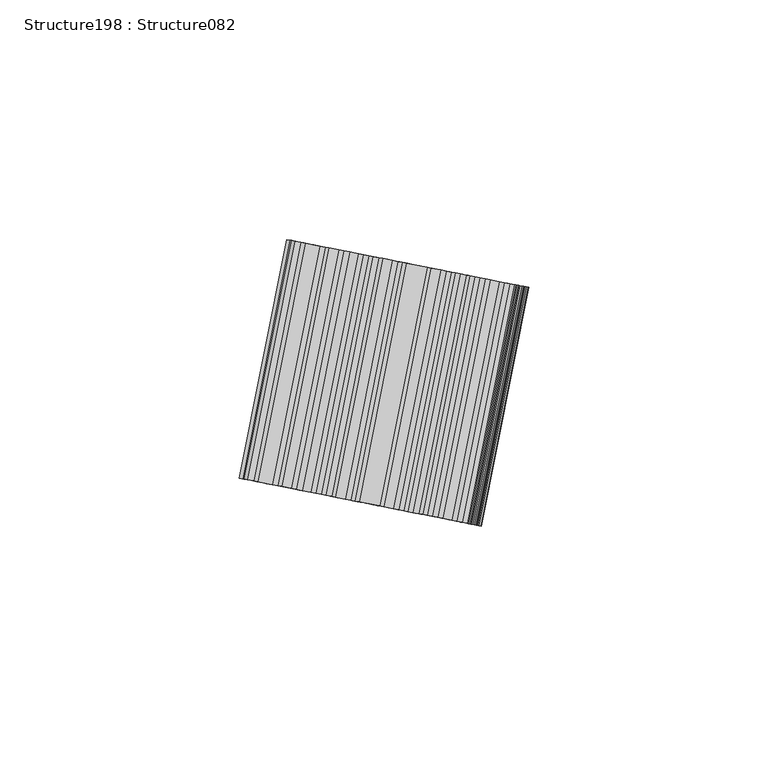
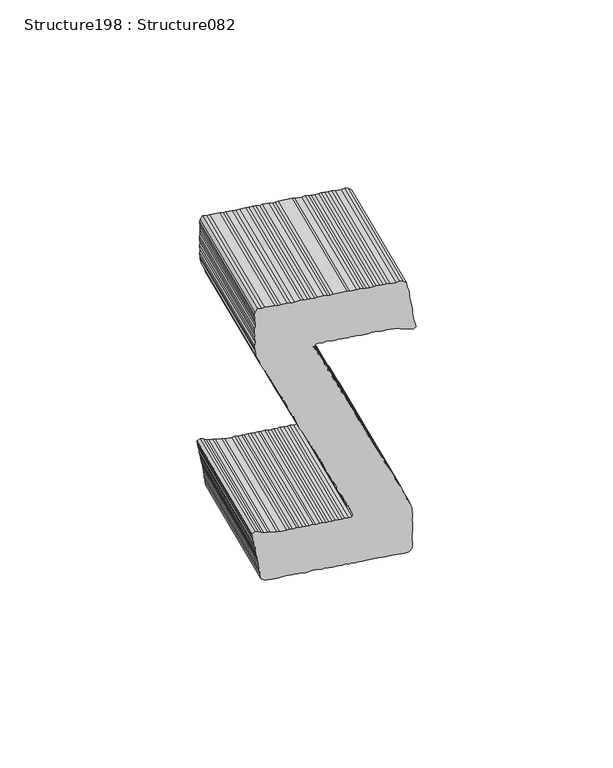
"""IFC4 building model written with IfcOpenShell, lengths in millimetres: proxy geometry, Structure198 : Structure082."""

import ifcopenshell
import ifcopenshell.guid

model = None  # the IFC model being written
_history = None  # IfcOwnerHistory: only IFC2X3 demands one
_inside = {}  # id of a spatial element -> (the spatial element, [elements in it])
_under = {}  # id of a project, library or spatial element -> (it, [spatial elements below it])
_declared = {}  # id of a project -> (the project, [libraries it declares])
_typed = {}  # id of a type object -> (the type object, [elements of that type])
_made_of = {}  # id of a material, layer set ... -> (it, [elements and type objects made of it])


def new_model(schema):
    """Start an empty IFC model of exactly this schema.

    Asked for "IFC4X3", IfcOpenShell would pick the latest addendum, in which some entities
    have other attributes; the version numbers below select the first issue.
    IFC2X3 requires an IfcOwnerHistory on every rooted entity: one is made here for all.
    """
    global model, _history
    if schema == "IFC4X3":
        model = ifcopenshell.file(schema_version=(4, 3, 0, 0))
    else:
        model = ifcopenshell.file(schema=schema)
    _inside.clear()
    _under.clear()
    _declared.clear()
    _typed.clear()
    _made_of.clear()
    _history = None
    if model.schema == "IFC2X3":
        org = make("IfcOrganization", Name="unknown")
        user = make(
            "IfcPersonAndOrganization",
            ThePerson=make("IfcPerson", FamilyName="unknown"),
            TheOrganization=org,
        )
        app = make(
            "IfcApplication",
            ApplicationDeveloper=org,
            Version="unknown",
            ApplicationFullName="unknown",
            ApplicationIdentifier="unknown",
        )
        _history = make(
            "IfcOwnerHistory",
            OwningUser=user,
            OwningApplication=app,
            ChangeAction="ADDED",
            CreationDate=0,
        )
    return model


def make(cls, **values):
    """One entity of the class cls with the attributes given. An attribute that is None is left unset."""
    return model.create_entity(
        cls, **{name: value for name, value in values.items() if value is not None}
    )


def rooted(cls, **values):
    """An entity with a GlobalId (a new one), such as an element, a storey or a relation."""
    return make(cls, GlobalId=ifcopenshell.guid.new(), OwnerHistory=_history, **values)


def si_unit(unit_type, name, prefix=None):
    """IfcSIUnit, for example si_unit("LENGTHUNIT", "METRE", prefix="MILLI")."""
    return make("IfcSIUnit", UnitType=unit_type, Prefix=prefix, Name=name)


def assignment(units):
    """IfcUnitAssignment: the units of a project."""
    return None if units is None else make("IfcUnitAssignment", Units=units)


def point(xyz):
    """IfcCartesianPoint."""
    return None if xyz is None else make("IfcCartesianPoint", Coordinates=xyz)


def direction(xyz):
    """IfcDirection."""
    return None if xyz is None else make("IfcDirection", DirectionRatios=xyz)


def frame(location, z_axis=None, x_axis=None):
    """IfcAxis2Placement3D, a coordinate frame: its origin and axes. An axis left out is left unset."""
    return make(
        "IfcAxis2Placement3D",
        Location=point(location),
        Axis=direction(z_axis),
        RefDirection=direction(x_axis),
    )


def origin():
    """The frame at (0, 0, 0) with its axes left unset."""
    return frame((0.0, 0.0, 0.0))


def place(relative_to, where):
    """IfcLocalPlacement: puts the frame where relative to a parent placement (None: the world)."""
    return make(
        "IfcLocalPlacement", PlacementRelTo=relative_to, RelativePlacement=where
    )


def context(
    kind, dimensions, precision=None, world=None, true_north=None, identifier=None
):
    """IfcGeometricRepresentationContext, for example the 3D "Model" context."""
    return make(
        "IfcGeometricRepresentationContext",
        ContextIdentifier=identifier,
        ContextType=kind,
        CoordinateSpaceDimension=dimensions,
        Precision=precision,
        WorldCoordinateSystem=world,
        TrueNorth=true_north,
    )


def project(units=None, contexts=None):
    """IfcProject with its units and contexts."""
    return rooted(
        "IfcProject",
        Name="project",
        RepresentationContexts=contexts,
        UnitsInContext=assignment(units),
    )


def spatial(cls, under=None, at=None, **own):
    """A site, building, storey or space (cls), placed at a placement, below another one or the project."""
    s = rooted(cls, ObjectPlacement=at, **own)
    if under is not None:
        _under.setdefault(under.id(), (under, []))[1].append(s)
    return s


def polyline(points):
    """IfcPolyline through the points."""
    return make("IfcPolyline", Points=[point(p) for p in points])


def outline(outer, holes=None, kind="AREA"):
    """IfcArbitraryClosedProfileDef: a profile drawn as a closed curve; with holes, ...WithVoids."""
    if holes is None:
        return make("IfcArbitraryClosedProfileDef", ProfileType=kind, OuterCurve=outer)
    return make(
        "IfcArbitraryProfileDefWithVoids",
        ProfileType=kind,
        OuterCurve=outer,
        InnerCurves=holes,
    )


def extrude(swept, where, along, depth):
    """IfcExtrudedAreaSolid: the profile swept, set in the frame where, extruded along a direction by depth."""
    return make(
        "IfcExtrudedAreaSolid",
        SweptArea=swept,
        Position=where,
        ExtrudedDirection=direction(along),
        Depth=depth,
    )


def shape(context_of_items, identifier, shape_type, items):
    """IfcShapeRepresentation: the items that make up one representation, for example the "Body"."""
    return make(
        "IfcShapeRepresentation",
        ContextOfItems=context_of_items,
        RepresentationIdentifier=identifier,
        RepresentationType=shape_type,
        Items=items,
    )


def source(mapping_origin, context_of_items, identifier, shape_type, items):
    """IfcRepresentationMap: a shape defined once, which mapped items show again and again."""
    return make(
        "IfcRepresentationMap",
        MappingOrigin=mapping_origin,
        MappedRepresentation=shape(context_of_items, identifier, shape_type, items),
    )


def transform(
    local_origin,
    x_axis=None,
    y_axis=None,
    z_axis=None,
    scale=None,
    scale2=None,
    scale3=None,
    uniform=True,
):
    """IfcCartesianTransformationOperator3D, or its non-uniform kind. x_axis, y_axis, z_axis: its Axis1, 2, 3."""
    if uniform:
        return make(
            "IfcCartesianTransformationOperator3D",
            Axis1=direction(x_axis),
            Axis2=direction(y_axis),
            LocalOrigin=point(local_origin),
            Scale=scale,
            Axis3=direction(z_axis),
        )
    return make(
        "IfcCartesianTransformationOperator3DnonUniform",
        Axis1=direction(x_axis),
        Axis2=direction(y_axis),
        LocalOrigin=point(local_origin),
        Scale=scale,
        Axis3=direction(z_axis),
        Scale2=scale2,
        Scale3=scale3,
    )


def mapped(mapping_source, mapping_target):
    """IfcMappedItem: shows the shape of a source again, moved by a transform."""
    return make(
        "IfcMappedItem", MappingSource=mapping_source, MappingTarget=mapping_target
    )


def made_of(thing, what):
    """Note that an element or type object is made of a material, layer set ...; save() writes the relation."""
    if what is not None:
        _made_of.setdefault(what.id(), (what, []))[1].append(thing)
    return thing


def element(
    cls,
    number,
    at=None,
    inside=None,
    cuts=None,
    type_object=None,
    material=None,
    context=None,
    identifier="Body",
    shape_type=None,
    held_by="IfcProductDefinitionShape",
    body=None,
    shapes=None,
    **own,
):
    """One element of the class cls, such as IfcWall. Its Tag is "e" and its number.

    at: its placement. inside: the storey or other place that contains it. cuts: it is an
    opening in that element (IfcRelVoidsElement). A single representation is given by context,
    identifier, shape_type and body (its items); several are given by shapes. held_by: the class
    of the entity that holds the representations. save() writes the other relations.
    """
    e = rooted(cls, Tag="e%d" % number, ObjectPlacement=at, **own)
    if body is not None:
        shapes = [shape(context, identifier, shape_type, body)]
    if shapes is not None:
        e.Representation = make(held_by, Representations=shapes)
    if inside is not None:
        _inside.setdefault(inside.id(), (inside, []))[1].append(e)
    if cuts is not None:
        rooted(
            "IfcRelVoidsElement", RelatingBuildingElement=cuts, RelatedOpeningElement=e
        )
    if type_object is not None:
        _typed.setdefault(type_object.id(), (type_object, []))[1].append(e)
    return made_of(e, material)


def aggregate(whole, parts):
    """IfcRelAggregates: a whole, such as a stair, and the parts it consists of."""
    return rooted("IfcRelAggregates", RelatingObject=whole, RelatedObjects=parts)


def save(model, path):
    """Write the relations noted so far, then the file.

    IfcRelAggregates (storeys below a building ...), IfcRelContainedInSpatialStructure (elements
    in a storey), IfcRelDefinesByType, IfcRelAssociatesMaterial and IfcRelDeclares: one each for
    every whole, place, type object, material and project.
    """
    for whole, parts in _under.values():
        aggregate(whole, parts)
    for where, things in _inside.values():
        rooted(
            "IfcRelContainedInSpatialStructure",
            RelatedElements=things,
            RelatingStructure=where,
        )
    for kind, things in _typed.values():
        rooted("IfcRelDefinesByType", RelatedObjects=things, RelatingType=kind)
    for what, things in _made_of.values():
        rooted("IfcRelAssociatesMaterial", RelatedObjects=things, RelatingMaterial=what)
    for by, libraries in _declared.values():
        rooted("IfcRelDeclares", RelatingContext=by, RelatedDefinitions=libraries)
    model.write(path)


def structure198_structure082_58b717cc(model_context):
    return source(origin(), model_context, "Body", "SweptSolid", [
        extrude(outline(polyline([(1.0465822, 0.0), (1.5142605, -1.0826543), (1.8028074, -2.1135614), (2.0909573, -3.1430563), (2.6061461, -4.0449016), (2.850272, -5.2548528), (3.1872117, -6.1093644), (3.6556848, -7.189106), (3.9440991, -8.2204987), (4.2203696, -8.9609175), (4.5094019, -9.991957), (4.9126595, -10.9618421), (5.4428175, -12.1509985), (5.8937621, -12.9403835), (6.1859717, -13.9741156), (6.525074, -14.8273918), (6.9391965, -16.0824248), (6.1536507, -17.5830856), (5.2962264, -17.9192304), (4.5730271, -18.4860339), (2.54318, -19.6456059), (0.6070291, -20.4512831), (-0.1826649, -20.9024043), (-1.1334764, -21.5922674), (-2.1003606, -21.9979086), (-2.6463697, -22.610192), (-3.6794395, -22.8999745), (-4.6780705, -23.770823), (-6.7263728, -24.6405679), (-8.4179121, -25.6068779), (-9.1900776, -26.3483557), (-10.1109961, -26.5740704), (-10.9971667, -27.3806748), (-12.0111634, -27.9599313), (-12.981048, -28.3603202), (-14.6704246, -29.3253948), (-15.7497691, -29.7952802), (-16.4113281, -30.4735728), (-17.3300838, -30.698052), (-18.32717, -31.5680181), (-19.2970547, -31.9684071), (-20.2482643, -32.6654639), (-21.2144415, -33.0637349), (-24.6003006, -34.9979434), (-25.6624256, -35.7583618), (-26.4039911, -36.028321), (-28.3232316, -37.1247078), (-29.1585823, -37.755579), (-31.7535117, -39.2379603), (-32.9476991, -39.7664846), (-34.315767, -39.2051539), (-35.0588773, -38.4294133), (-35.508057, -37.643118), (-35.862216, -36.4980732), (-36.4931749, -35.658265), (-37.0083638, -34.7564197), (-37.5073921, -34.1432538), (-39.0547235, -31.4346283), (-39.3428734, -30.4051335), (-40.2114716, -29.4097246), (-40.6011725, -28.7275476), (-41.0176342, -27.4734411), (-41.534588, -26.5685062), (-41.9836354, -24.7351432), (-42.0347195, -23.8595278), (-42.0320719, -22.81758), (-42.2105855, -21.7188976), (-42.4503427, -20.5130072), (-42.3214126, -19.6878151), (-42.5655386, -18.4778639), (-42.7883853, -17.5626831), (-42.5479661, -16.6758505), (-42.8533791, -15.3521594), (-42.7910767, -13.3709256), (-43.1920839, -12.4042626), (-43.3072798, -10.3691192), (-43.1926575, -9.2627947), (-43.3049854, -8.2799713), (-43.3048529, -7.2329036), (-43.3031757, -6.1849535), (-43.7742525, -5.1042406), (-43.6423219, -4.2843008), (-43.7083751, -3.1213743), (-43.770942, -1.9609638), (-43.9511768, 0.1837271), (-44.0597094, 1.164211), (-44.1739788, 2.150433), (-44.0452699, 2.9709912), (-44.3991199, 4.1162124), (-44.2211359, 5.1116214), (-44.2871891, 6.2745479), (-44.5119773, 7.1931272), (-44.5100798, 8.2371052), (-44.5581635, 9.1074684), (-44.7365893, 10.2016932), (-44.6869601, 11.4311143), (-44.8652094, 12.5250302), (-44.9147487, 13.401528), (-45.2062972, 14.4290814), (-45.2025896, 15.4777816), (-45.2685551, 16.6362505), (-45.2040456, 18.6207942), (-45.4739171, 19.3579021), (-45.4921955, 20.6968712), (-45.4305992, 21.6327588), (-45.6538426, 22.5522205), (-45.7675828, 23.534647), (-45.781007, 24.8694227), (-45.898189, 25.8564395), (-46.0723338, 26.9510609), (-45.8294878, 27.8343626), (-46.1845292, 28.9809521), (-46.166162, 30.7858781), (-46.2338924, 31.9474367), (-46.5861099, 33.0890829), (-46.5859775, 34.1361505), (-46.409935, 35.134958), (-46.8111186, 36.1019299), (-46.8139866, 37.1542499), (-46.6973341, 38.2613244), (-47.1038578, 39.2297534), (-46.9729862, 40.051547), (-47.1513232, 41.1499203), (-47.1008563, 42.3728537), (-47.2148614, 43.3543093), (-47.1498665, 44.2921382), (-47.1473955, 45.334395), (-48.2286368, 45.9194332), (-49.2612212, 45.6295185), (-50.1475683, 44.823223), (-51.1789169, 44.5340141), (-51.9683019, 44.0830695), (-52.7424976, 43.3408416), (-53.5321916, 42.8897205), (-54.6769274, 42.535738), (-55.2911082, 42.037769), (-56.1252672, 41.4083981), (-57.1426624, 40.8272002), (-58.0612417, 40.602412), (-58.7875739, 40.0403753), (-59.9155756, 39.3959922), (-60.5251229, 38.8949332), (-62.4462172, 37.7974874), (-63.5878633, 37.4452699), (-65.1684871, 36.5423216), (-65.9426828, 35.8000937), (-66.7323767, 35.3489726), (-67.9895728, 34.9307459), (-68.6497635, 34.2536447), (-70.2285334, 33.3517554), (-71.0991615, 32.2561187), (-71.7582932, 31.5771638), (-72.598807, 30.9503094), (-73.3209914, 30.3824465), (-73.9700082, 29.4203739), (-75.1444613, 29.6427788), (-75.5472774, 30.6133258), (-75.6599143, 31.5959728), (-75.9491231, 32.6273214), (-76.4825907, 33.8186848), (-76.756345, 34.5625899), (-77.3979043, 35.6856483), (-77.8037657, 36.6565046), (-77.9611769, 37.4578568), (-78.7208883, 39.5739343), (-78.9457653, 40.488365), (-79.5289047, 41.5091587), (-79.9296029, 42.4759982), (-80.2196065, 43.5044341), (-80.3809006, 44.3125834), (-80.7963034, 45.5648361), (-80.2833642, 46.7651146), (-79.3967969, 47.567438), (-78.3678312, 47.8593834), (-76.6744382, 48.8267524), (-75.9003312, 49.5648317), (-74.8205457, 50.0325103), (-73.9810907, 50.6612185), (-73.0807902, 51.1755248), (-72.3374587, 51.4510005), (-71.1465807, 51.9846005), (-70.2428816, 52.5008483), (-69.5166819, 53.0623996), (-68.6809345, 53.6889898), (-67.5989862, 54.157904), (-65.7952956, 55.1882816), (-65.1807614, 55.6885014), (-61.3475326, 57.8782746), (-60.4939035, 58.216759), (-59.6394795, 58.558156), (-58.7510585, 59.3615383), (-56.9476769, 60.3917395), (-56.1430139, 60.5555496), (-55.1405878, 61.4240586), (-54.3508938, 61.8751798), (-53.2729619, 62.3417995), (-52.4335071, 62.9705076), (-50.7273078, 63.64933), (-49.598997, 64.2938897), (-48.7584832, 64.9207441), (-46.9551016, 65.9509453), (-46.2165365, 66.2261567), (-45.3265707, 67.0304216), (-42.619181, 68.5770471), (-41.7023666, 68.8049248), (-40.7002495, 69.6732574), (-39.441156, 69.0422977), (-38.8785454, 68.3171129), (-38.4091899, 67.2358265), (-37.9608926, 66.4510759), (-37.5601944, 65.4842364), (-36.977055, 64.4634427), (-36.3017187, 63.8063416), (-35.7874124, 62.9060411), (-35.3152329, 61.8198115), (-34.6912021, 60.9871096), (-34.0795369, 59.3912967), (-33.2721825, 58.5030958), (-32.8024739, 57.4211915), (-32.5329115, 56.6839071), (-31.9022619, 54.7944715), (-31.7914347, 52.7633889), (-31.3883969, 51.8003446), (-31.3716193, 50.4596987), (-31.325168, 49.5929105), (-31.4349369, 48.4766555), (-31.3239773, 47.4926405), (-31.3219471, 46.4468083), (-31.0344151, 45.4169606), (-31.2123991, 44.4215517), (-30.8094504, 43.4514902), (-30.7909955, 42.1122121), (-30.6298339, 41.3035774), (-30.5666487, 40.1463887), (-30.5193598, 39.2731128), (-30.3897237, 38.0039047), (-30.6341146, 37.1197207), (-30.2926298, 36.2608393), (-30.1667452, 34.9903077), (-30.3430967, 33.9913238), (-30.2305924, 33.0081913), (-30.0513729, 31.9082732), (-29.9881436, 30.75029), (-29.5864745, 28.7366034), (-29.9428403, 27.7880427), (-29.6508071, 26.7546195), (-29.5383027, 25.7714871), (-29.5217893, 24.4356076), (-29.3610688, 23.6291797), (-29.1849822, 22.5340284), (-29.2968694, 21.418612), (-29.1362365, 20.6166416), (-29.1379138, 19.5686915), (-29.1378698, 18.5213149), (-28.9575025, 17.4236916), (-29.0713311, 16.3116737), (-28.7347005, 15.4569856), (-28.8321922, 14.0559796), (-28.6061682, 13.1381062), (-28.6037413, 12.0879931), (-28.5396296, 10.928465), (-28.4291554, 9.9445826), (-28.4934433, 9.0141238), (-28.2506856, 7.8029812), (-28.2523628, 6.7550311), (-28.040646, 5.0774452), (-27.8501639, 3.6967041), (-27.960992, 2.5794341), (-27.8484877, 0.5497194), (-27.5760125, -0.1883598), (-27.737086, -1.4744784), (-27.5113276, -2.39906), (-27.6234349, -3.5105042), (-27.2208829, -4.4762847), (-27.1102323, -5.4604761), (-27.2860984, -7.5061747), (-27.0463411, -8.7120651), (-26.9794055, -9.8765363), (-26.9807738, -10.92431), (-26.6402592, -11.7771891), (-26.8049078, -13.0649402), (-26.5800755, -15.030896), (-26.4152953, -15.8415613), (-25.8054391, -16.386908), (-24.72583, -15.9189205), (-23.7725025, -15.2255711), (-22.9187408, -14.8866013), (-22.0190582, -14.3726479), (-21.0669665, -13.6800045), (-20.1457834, -13.4561876), (-19.3116686, -12.8260225), (-18.5667046, -12.5541218), (-17.6188935, -11.8590065), (-16.8917225, -11.2948514), (-15.6331585, -10.8783021), (-15.0864871, -10.2635913), (-14.0084227, -9.7964862), (-13.1047237, -9.2802384), (-12.267255, -8.6530746), (-11.2348475, -8.3657195), (-10.6241084, -7.8631602), (-9.4280673, -7.3335769), (-8.7686267, -6.6544455), (-7.7368371, -6.3674434), (-5.9316017, -5.3361833), (-5.1581559, -4.5919252), (-3.5981502, -3.4003853), (-2.9834395, -2.9004745), (-1.9211379, -2.1403649), (-1.371246, -1.5348784), (-0.8394548, -0.6287082), (0.0, 0.0), (1.0465822, 0.0)])), frame((-1845.4685864, 234834.727126, 404.8484925), z_axis=(0.1946622229639412, 0.9808703374813295, 0.0), x_axis=(-0.8516955016572499, 0.1690263568033965, -0.49602909507666604)), (0.0, 0.0, 1.0), 50.8),
    ])


if __name__ == "__main__":
    model = new_model("IFC4")
    model_context = context("Model", 3, world=origin())
    ifc_project = project(units=[si_unit("LENGTHUNIT", "METRE", prefix="MILLI")], contexts=[model_context])
    site = spatial("IfcSite", under=ifc_project)
    building = spatial("IfcBuilding", under=site)
    placement = place(None, origin())
    structure198_structure082_shape = structure198_structure082_58b717cc(model_context)
    element("IfcBuildingElementProxy", 1, Name="Structure198 : Structure082", ObjectType="Structure198 : Structure082", at=placement, inside=building, context=model_context, shape_type="MappedRepresentation", body=[
        mapped(structure198_structure082_shape, transform((0.0, 0.0, 0.0), x_axis=(1.0, 0.0, 0.0), y_axis=(0.0, 1.0, 0.0), z_axis=(0.0, 0.0, 1.0))),
    ])
    save(model, "model.ifc")

# Revit data of these elements
# Type "Structure198 : Structure082"
#   NameOverride = "Structure082"
# Element 1 (IfcBuildingElementProxy, "Structure198 : Structure082")
#   Materials on its faces: "BRUSHED ALUMINUM LETTERING"
# Materials
#   "BRUSHED ALUMINUM LETTERING": class "Unassigned", colour RGB 169 181 186, transparency 0, Cost = 0
